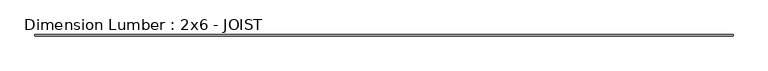
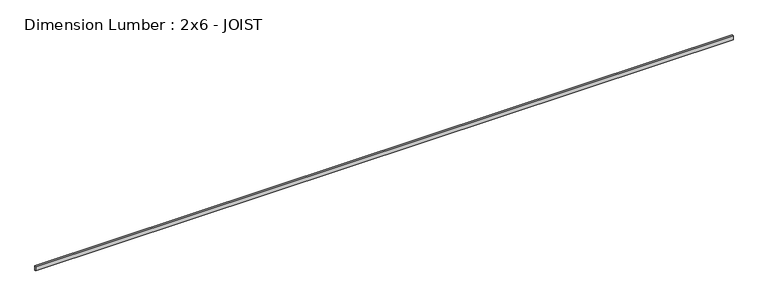
"""IFC4 building model written with IfcOpenShell, lengths in millimetres: beam geometry, Dimension Lumber : 2x6 - JOIST."""

import ifcopenshell
import ifcopenshell.guid

model = None  # the IFC model being written
_history = None  # IfcOwnerHistory: only IFC2X3 demands one
_inside = {}  # id of a spatial element -> (the spatial element, [elements in it])
_under = {}  # id of a project, library or spatial element -> (it, [spatial elements below it])
_declared = {}  # id of a project -> (the project, [libraries it declares])
_typed = {}  # id of a type object -> (the type object, [elements of that type])
_made_of = {}  # id of a material, layer set ... -> (it, [elements and type objects made of it])


def new_model(schema):
    """Start an empty IFC model of exactly this schema.

    Asked for "IFC4X3", IfcOpenShell would pick the latest addendum, in which some entities
    have other attributes; the version numbers below select the first issue.
    IFC2X3 requires an IfcOwnerHistory on every rooted entity: one is made here for all.
    """
    global model, _history
    if schema == "IFC4X3":
        model = ifcopenshell.file(schema_version=(4, 3, 0, 0))
    else:
        model = ifcopenshell.file(schema=schema)
    _inside.clear()
    _under.clear()
    _declared.clear()
    _typed.clear()
    _made_of.clear()
    _history = None
    if model.schema == "IFC2X3":
        org = make("IfcOrganization", Name="unknown")
        user = make(
            "IfcPersonAndOrganization",
            ThePerson=make("IfcPerson", FamilyName="unknown"),
            TheOrganization=org,
        )
        app = make(
            "IfcApplication",
            ApplicationDeveloper=org,
            Version="unknown",
            ApplicationFullName="unknown",
            ApplicationIdentifier="unknown",
        )
        _history = make(
            "IfcOwnerHistory",
            OwningUser=user,
            OwningApplication=app,
            ChangeAction="ADDED",
            CreationDate=0,
        )
    return model


def make(cls, **values):
    """One entity of the class cls with the attributes given. An attribute that is None is left unset."""
    return model.create_entity(
        cls, **{name: value for name, value in values.items() if value is not None}
    )


def rooted(cls, **values):
    """An entity with a GlobalId (a new one), such as an element, a storey or a relation."""
    return make(cls, GlobalId=ifcopenshell.guid.new(), OwnerHistory=_history, **values)


def si_unit(unit_type, name, prefix=None):
    """IfcSIUnit, for example si_unit("LENGTHUNIT", "METRE", prefix="MILLI")."""
    return make("IfcSIUnit", UnitType=unit_type, Prefix=prefix, Name=name)


def assignment(units):
    """IfcUnitAssignment: the units of a project."""
    return None if units is None else make("IfcUnitAssignment", Units=units)


def point(xyz):
    """IfcCartesianPoint."""
    return None if xyz is None else make("IfcCartesianPoint", Coordinates=xyz)


def direction(xyz):
    """IfcDirection."""
    return None if xyz is None else make("IfcDirection", DirectionRatios=xyz)


def frame(location, z_axis=None, x_axis=None):
    """IfcAxis2Placement3D, a coordinate frame: its origin and axes. An axis left out is left unset."""
    return make(
        "IfcAxis2Placement3D",
        Location=point(location),
        Axis=direction(z_axis),
        RefDirection=direction(x_axis),
    )


def origin():
    """The frame at (0, 0, 0) with its axes left unset."""
    return frame((0.0, 0.0, 0.0))


def place(relative_to, where):
    """IfcLocalPlacement: puts the frame where relative to a parent placement (None: the world)."""
    return make(
        "IfcLocalPlacement", PlacementRelTo=relative_to, RelativePlacement=where
    )


def context(
    kind, dimensions, precision=None, world=None, true_north=None, identifier=None
):
    """IfcGeometricRepresentationContext, for example the 3D "Model" context."""
    return make(
        "IfcGeometricRepresentationContext",
        ContextIdentifier=identifier,
        ContextType=kind,
        CoordinateSpaceDimension=dimensions,
        Precision=precision,
        WorldCoordinateSystem=world,
        TrueNorth=true_north,
    )


def project(units=None, contexts=None):
    """IfcProject with its units and contexts."""
    return rooted(
        "IfcProject",
        Name="project",
        RepresentationContexts=contexts,
        UnitsInContext=assignment(units),
    )


def spatial(cls, under=None, at=None, **own):
    """A site, building, storey or space (cls), placed at a placement, below another one or the project."""
    s = rooted(cls, ObjectPlacement=at, **own)
    if under is not None:
        _under.setdefault(under.id(), (under, []))[1].append(s)
    return s


def polyline(points):
    """IfcPolyline through the points."""
    return make("IfcPolyline", Points=[point(p) for p in points])


def outline(outer, holes=None, kind="AREA"):
    """IfcArbitraryClosedProfileDef: a profile drawn as a closed curve; with holes, ...WithVoids."""
    if holes is None:
        return make("IfcArbitraryClosedProfileDef", ProfileType=kind, OuterCurve=outer)
    return make(
        "IfcArbitraryProfileDefWithVoids",
        ProfileType=kind,
        OuterCurve=outer,
        InnerCurves=holes,
    )


def extrude(swept, where, along, depth):
    """IfcExtrudedAreaSolid: the profile swept, set in the frame where, extruded along a direction by depth."""
    return make(
        "IfcExtrudedAreaSolid",
        SweptArea=swept,
        Position=where,
        ExtrudedDirection=direction(along),
        Depth=depth,
    )


def shape(context_of_items, identifier, shape_type, items):
    """IfcShapeRepresentation: the items that make up one representation, for example the "Body"."""
    return make(
        "IfcShapeRepresentation",
        ContextOfItems=context_of_items,
        RepresentationIdentifier=identifier,
        RepresentationType=shape_type,
        Items=items,
    )


def source(mapping_origin, context_of_items, identifier, shape_type, items):
    """IfcRepresentationMap: a shape defined once, which mapped items show again and again."""
    return make(
        "IfcRepresentationMap",
        MappingOrigin=mapping_origin,
        MappedRepresentation=shape(context_of_items, identifier, shape_type, items),
    )


def transform(
    local_origin,
    x_axis=None,
    y_axis=None,
    z_axis=None,
    scale=None,
    scale2=None,
    scale3=None,
    uniform=True,
):
    """IfcCartesianTransformationOperator3D, or its non-uniform kind. x_axis, y_axis, z_axis: its Axis1, 2, 3."""
    if uniform:
        return make(
            "IfcCartesianTransformationOperator3D",
            Axis1=direction(x_axis),
            Axis2=direction(y_axis),
            LocalOrigin=point(local_origin),
            Scale=scale,
            Axis3=direction(z_axis),
        )
    return make(
        "IfcCartesianTransformationOperator3DnonUniform",
        Axis1=direction(x_axis),
        Axis2=direction(y_axis),
        LocalOrigin=point(local_origin),
        Scale=scale,
        Axis3=direction(z_axis),
        Scale2=scale2,
        Scale3=scale3,
    )


def mapped(mapping_source, mapping_target):
    """IfcMappedItem: shows the shape of a source again, moved by a transform."""
    return make(
        "IfcMappedItem", MappingSource=mapping_source, MappingTarget=mapping_target
    )


def made_of(thing, what):
    """Note that an element or type object is made of a material, layer set ...; save() writes the relation."""
    if what is not None:
        _made_of.setdefault(what.id(), (what, []))[1].append(thing)
    return thing


def element(
    cls,
    number,
    at=None,
    inside=None,
    cuts=None,
    type_object=None,
    material=None,
    context=None,
    identifier="Body",
    shape_type=None,
    held_by="IfcProductDefinitionShape",
    body=None,
    shapes=None,
    **own,
):
    """One element of the class cls, such as IfcWall. Its Tag is "e" and its number.

    at: its placement. inside: the storey or other place that contains it. cuts: it is an
    opening in that element (IfcRelVoidsElement). A single representation is given by context,
    identifier, shape_type and body (its items); several are given by shapes. held_by: the class
    of the entity that holds the representations. save() writes the other relations.
    """
    e = rooted(cls, Tag="e%d" % number, ObjectPlacement=at, **own)
    if body is not None:
        shapes = [shape(context, identifier, shape_type, body)]
    if shapes is not None:
        e.Representation = make(held_by, Representations=shapes)
    if inside is not None:
        _inside.setdefault(inside.id(), (inside, []))[1].append(e)
    if cuts is not None:
        rooted(
            "IfcRelVoidsElement", RelatingBuildingElement=cuts, RelatedOpeningElement=e
        )
    if type_object is not None:
        _typed.setdefault(type_object.id(), (type_object, []))[1].append(e)
    return made_of(e, material)


def aggregate(whole, parts):
    """IfcRelAggregates: a whole, such as a stair, and the parts it consists of."""
    return rooted("IfcRelAggregates", RelatingObject=whole, RelatedObjects=parts)


def save(model, path):
    """Write the relations noted so far, then the file.

    IfcRelAggregates (storeys below a building ...), IfcRelContainedInSpatialStructure (elements
    in a storey), IfcRelDefinesByType, IfcRelAssociatesMaterial and IfcRelDeclares: one each for
    every whole, place, type object, material and project.
    """
    for whole, parts in _under.values():
        aggregate(whole, parts)
    for where, things in _inside.values():
        rooted(
            "IfcRelContainedInSpatialStructure",
            RelatedElements=things,
            RelatingStructure=where,
        )
    for kind, things in _typed.values():
        rooted("IfcRelDefinesByType", RelatedObjects=things, RelatingType=kind)
    for what, things in _made_of.values():
        rooted("IfcRelAssociatesMaterial", RelatedObjects=things, RelatingMaterial=what)
    for by, libraries in _declared.values():
        rooted("IfcRelDeclares", RelatingContext=by, RelatedDefinitions=libraries)
    model.write(path)


def dimension_lumber_2x6_joist_10b0e315(model_context):
    return source(origin(), model_context, "Body", "SweptSolid", [
        extrude(outline(polyline([(10526.5600685, 19.05), (10526.5600685, -19.05), (-10526.5600685, -19.05), (-10526.5600685, 19.05), (10526.5600685, 19.05)])), frame((0.0, 0.0, -66.675), z_axis=(0.0, 0.0, 1.0), x_axis=(1.0, 0.0, 0.0)), (0.0, 0.0, 1.0), 133.35),
    ])


if __name__ == "__main__":
    model = new_model("IFC4")
    model_context = context("Model", 3, world=origin())
    ifc_project = project(units=[si_unit("LENGTHUNIT", "METRE", prefix="MILLI")], contexts=[model_context])
    site = spatial("IfcSite", under=ifc_project)
    building = spatial("IfcBuilding", under=site)
    placement = place(None, origin())
    dimension_lumber_2x6_joist_shape = dimension_lumber_2x6_joist_10b0e315(model_context)
    element("IfcBeam", 1, ObjectType="Dimension Lumber : 2x6 - JOIST", at=placement, inside=building, context=model_context, shape_type="MappedRepresentation", body=[
        mapped(dimension_lumber_2x6_joist_shape, transform((0.0, 0.0, 0.0), x_axis=(1.0, 0.0, 0.0), y_axis=(0.0, 1.0, 0.0), z_axis=(0.0, 0.0, 1.0))),
    ])
    save(model, "model.ifc")

# Revit data of these elements
# Type "Dimension Lumber : 2x6 - JOIST"
#   Assembly Code = "B10"
#   A = 0.0963889 SF
#   Length [instance default] = 5' - 0"
#   b = 0' - 1 1/2"
#   d = 0' - 5 1/4"
#   Structural Material = 2X10 JOISTS
# Element 1 (IfcBeam, "Dimension Lumber : 2x6 - JOIST")
#   Materials on its faces: "2X10 JOISTS"
# Materials
#   "2X10 JOISTS": class "Wood", colour RGB 234 198 147, transparency 0, Description = "Pinus Echinata", Cost = 0
